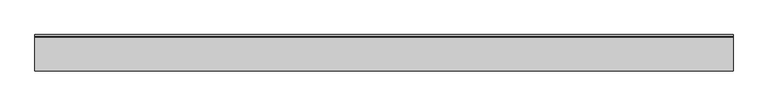
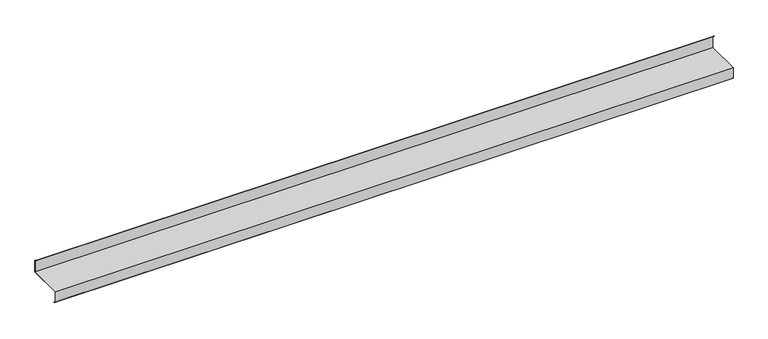
"""IFC4 building model written with IfcOpenShell, lengths in millimetres: proxy geometry, Generic Models 7:Generic Models 1:337419:Generic Models 1:337419 : Generic Models 7:Generic Models 1:337419:12 : Generic Models 7:Generic Models 1:337419:Generic Models 1:337419 : Generic Models 7:Generic Models 1:337419:301336."""

from ifc_helpers import new_model, si_unit, frame, origin, place, context, project, spatial, polyline, outline, extrude, source, transform, mapped, element, save


def generic_models_03751d16(model_context):
    return source(origin(), model_context, "Body", "SweptSolid", [
        extrude(outline(polyline([(-567932.6413841, 7351.7125), (-568183.8632591, 7351.7125), (-568183.8632591, 7276.411086), (-568170.0763026, 7264.8424559), (-568172.0482374, 7262.870521), (-568186.6413841, 7275.115625), (-568186.6413841, 7354.490625), (-567935.4195091, 7354.490625), (-567935.4195091, 7436.142039), (-567949.0202751, 7447.5544367), (-567947.0483402, 7449.5263716), (-567932.6413841, 7437.4375), (-567932.6413841, 7351.7125)])), frame((591306.0367242, 0.0, 0.0), z_axis=(1.0, 0.0, 0.0), x_axis=(0.0, 1.0, 0.0)), (0.0, 0.0, 1.0), 4876.8),
    ])


if __name__ == "__main__":
    model = new_model("IFC4")
    model_context = context("Model", 3, world=origin())
    ifc_project = project(units=[si_unit("LENGTHUNIT", "METRE", prefix="MILLI")], contexts=[model_context])
    site = spatial("IfcSite", under=ifc_project)
    building = spatial("IfcBuilding", under=site)
    placement = place(None, origin())
    generic_models_shape = generic_models_03751d16(model_context)
    element("IfcBuildingElementProxy", 1, Name="Generic Models 7:Generic Models 1:337419:Generic Models 1:337419 : Generic Models 7:Generic Models 1:337419:12 : Generic Models 7:Generic Models 1:337419:Generic Models 1:337419 : Generic Models 7:Generic Models 1:337419:301336", ObjectType="Generic Models 7:Generic Models 1:337419:Generic Models 1:337419 : Generic Models 7:Generic Models 1:337419:12 : Generic Models 7:Generic Models 1:337419:Generic Models 1:337419 : Generic Models 7:Generic Models 1:337419:301336", at=placement, inside=building, context=model_context, shape_type="MappedRepresentation", body=[
        mapped(generic_models_shape, transform((0.0, 0.0, 0.0), x_axis=(1.0, 0.0, 0.0), y_axis=(0.0, 1.0, 0.0), z_axis=(0.0, 0.0, 1.0))),
    ])
    save(model, "model.ifc")

# Revit data of these elements
# Type "Generic Models 7:Generic Models 1:337419:Generic Models 1:337419 : Generic Models 7:Generic Models 1:337419:12 : Generic Models 7:Generic Models 1:337419:Generic Models 1:337419 : Generic Models 7:Generic Models 1:337419:301336"
#   NameOverride = "Generic Models 7:Generic Models 1:337419:Generic Models 1:337419 : Generic Models 7:Generic Models 1:337419:301336"
#   ObjectTypeOverride = "Generic Models 1:337419 : Generic Models 7:Generic Models 1:337419"
#   Reference = "Generic Models 1"
#   Tag = "301336"
# Element 1 (IfcBuildingElementProxy, "Generic Models 7:Generic Models 1:337419:Generic Models 1:337419 : Generic Models 7:Generic Models 1:337419:12 : Generic Models 7:Generic Models 1:337419:Generic Models 1:337419 : Generic Models 7:Generic Models 1:337419:301336")
#   Materials on its faces: "'ZEE' SECTION (8.0x3.5Z - SEE STRUCT. DWGS)"
# Materials
#   "'ZEE' SECTION (8.0x3.5Z - SEE STRUCT. DWGS)": class "Unassigned", colour RGB 210 209 208, transparency 0, Keynote = "M05121300.02", Cost = 0
